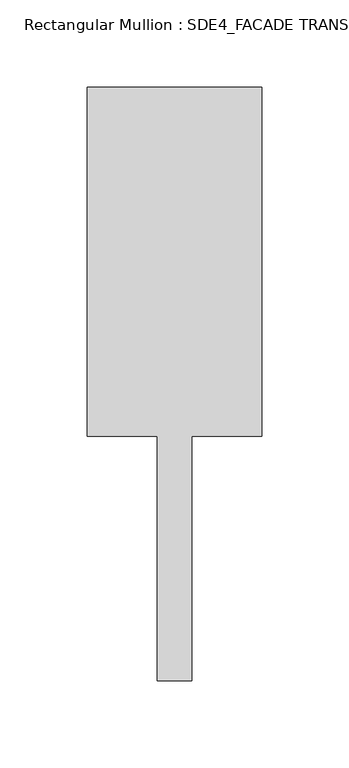
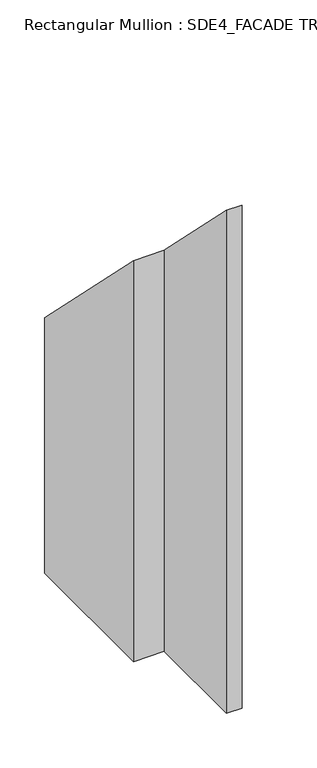
"""IFC4 building model written with IfcOpenShell, lengths in millimetres: member geometry, Rectangular Mullion : SDE4_FACADE TRANSOM TYPE 1."""

from ifc_helpers import new_model, si_unit, origin, place, context, project, spatial, faceted_brep, source, transform, mapped, element, save


def rectangular_mullion_sde4_facade_transom_type_1_5f2b7471(model_context):
    return source(origin(), model_context, "Body", "Brep", [
        faceted_brep([(50.0, 132.5, -482.5), (50.0, -67.5, -482.5), (10.0, -67.5, -482.5), (10.0, -207.5, -482.5), (-10.0, -207.5, -482.5), (-10.0, -67.5, -482.5), (-50.0, -67.5, -482.5), (-50.0, 132.5, -482.5), (-50.0, 132.5, -132.5), (50.0, 132.5, -132.5), (-50.0, -67.5, 67.5), (-10.0, -67.5, 67.5), (-10.0, -207.5, 207.5), (10.0, -207.5, 207.5), (10.0, -67.5, 67.5), (50.0, -67.5, 67.5)], [[[0, 1, 2, 3, 4, 5, 6, 7]], [[8, 9, 0, 7]], [[10, 8, 7, 6]], [[11, 10, 6, 5]], [[12, 11, 5, 4]], [[13, 12, 4, 3]], [[14, 13, 3, 2]], [[15, 14, 2, 1]], [[9, 15, 1, 0]], [[9, 8, 10, 11, 12, 13, 14, 15]]]),
    ])


if __name__ == "__main__":
    model = new_model("IFC4")
    model_context = context("Model", 3, world=origin())
    ifc_project = project(units=[si_unit("LENGTHUNIT", "METRE", prefix="MILLI")], contexts=[model_context])
    site = spatial("IfcSite", under=ifc_project)
    building = spatial("IfcBuilding", under=site)
    placement = place(None, origin())
    rectangular_mullion_sde4_facade_transom_type_1_shape = rectangular_mullion_sde4_facade_transom_type_1_5f2b7471(model_context)
    element("IfcMember", 1, ObjectType="Rectangular Mullion : SDE4_FACADE TRANSOM TYPE 1", at=placement, inside=building, context=model_context, shape_type="MappedRepresentation", body=[
        mapped(rectangular_mullion_sde4_facade_transom_type_1_shape, transform((0.0, 0.0, 0.0), x_axis=(1.0, 0.0, 0.0), y_axis=(0.0, 1.0, 0.0), z_axis=(0.0, 0.0, 1.0))),
    ])
    save(model, "model.ifc")

# Revit data of these elements
# Type "Rectangular Mullion : SDE4_FACADE TRANSOM TYPE 1"
#   built-in parameter 1007322 = 1.11549 (stored number, unit not read)
#   built-in parameter 1007321 = 0.164042 (stored number, unit not read)
#   built-in parameter 1007320 = 0.164042 (stored number, unit not read)
